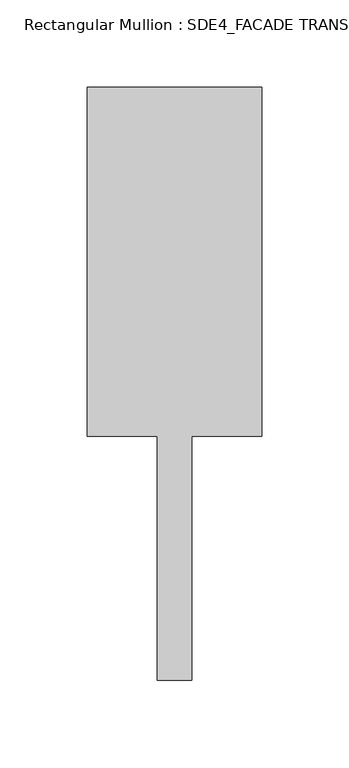
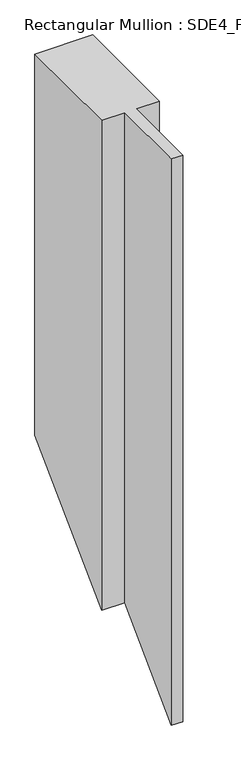
"""IFC4 building model written with IfcOpenShell, lengths in millimetres: member geometry, Rectangular Mullion : SDE4_FACADE TRANSOM TYPE 1."""

from ifc_helpers import new_model, si_unit, origin, place, context, project, spatial, faceted_brep, source, transform, mapped, element, save


def rectangular_mullion_sde4_facade_transom_type_1_20750b05(model_context):
    return source(origin(), model_context, "Body", "Brep", [
        faceted_brep([(50.0, 132.5, 0.0), (-50.0, 132.5, 0.0), (-50.0, -67.5, 0.0), (-10.0, -67.5, 0.0), (-10.0, -207.5, 0.0), (10.0, -207.5, 0.0), (10.0, -67.5, 0.0), (50.0, -67.5, 0.0), (50.0, 132.5, -698.0990258), (-50.0, 132.5, -698.0990258), (-50.0, -67.5, -898.0990258), (-10.0, -67.5, -898.0990258), (-10.0, -207.5, -1038.0990258), (10.0, -207.5, -1038.0990258), (10.0, -67.5, -898.0990258), (50.0, -67.5, -898.0990258)], [[[0, 1, 2, 3, 4, 5, 6, 7]], [[1, 0, 8, 9]], [[2, 1, 9, 10]], [[3, 2, 10, 11]], [[4, 3, 11, 12]], [[5, 4, 12, 13]], [[6, 5, 13, 14]], [[7, 6, 14, 15]], [[0, 7, 15, 8]], [[8, 15, 14, 13, 12, 11, 10, 9]]]),
    ])


if __name__ == "__main__":
    model = new_model("IFC4")
    model_context = context("Model", 3, world=origin())
    ifc_project = project(units=[si_unit("LENGTHUNIT", "METRE", prefix="MILLI")], contexts=[model_context])
    site = spatial("IfcSite", under=ifc_project)
    building = spatial("IfcBuilding", under=site)
    placement = place(None, origin())
    rectangular_mullion_sde4_facade_transom_type_1_shape = rectangular_mullion_sde4_facade_transom_type_1_20750b05(model_context)
    element("IfcMember", 1, ObjectType="Rectangular Mullion : SDE4_FACADE TRANSOM TYPE 1", at=placement, inside=building, context=model_context, shape_type="MappedRepresentation", body=[
        mapped(rectangular_mullion_sde4_facade_transom_type_1_shape, transform((0.0, 0.0, 0.0), x_axis=(1.0, 0.0, 0.0), y_axis=(0.0, 1.0, 0.0), z_axis=(0.0, 0.0, 1.0))),
    ])
    save(model, "model.ifc")

# Revit data of these elements
# Type "Rectangular Mullion : SDE4_FACADE TRANSOM TYPE 1"
#   built-in parameter 1007322 = 1.11549 (stored number, unit not read)
#   built-in parameter 1007321 = 0.164042 (stored number, unit not read)
#   built-in parameter 1007320 = 0.164042 (stored number, unit not read)
